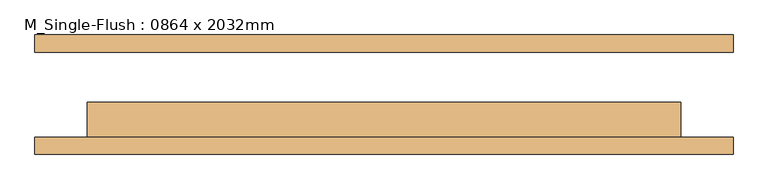
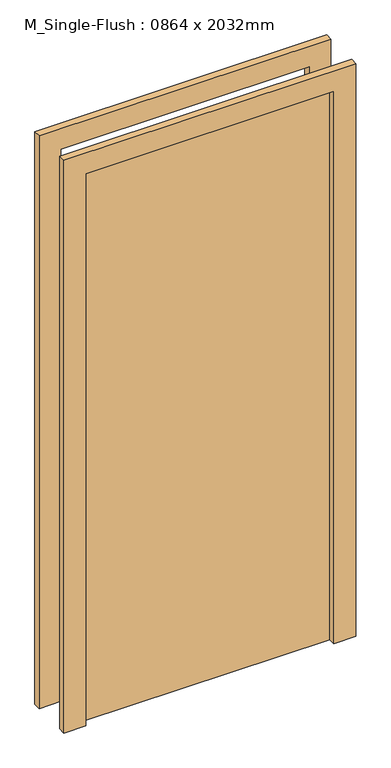
"""IFC4 building model written with IfcOpenShell, lengths in millimetres: door geometry, M_Single-Flush : 0864 x 2032mm."""

from ifc_helpers import new_model, si_unit, frame, origin, origin_with_axes, place, context, project, spatial, polyline, outline, extrude, source, transform, mapped, element, save


def m_single_flush_0864_x_2032mm_954ee019(model_context):
    return source(origin(), model_context, "Body", "SweptSolid", [
        extrude(outline(polyline([(2108.0, -508.0), (0.0, -508.0), (0.0, -432.0), (2032.0, -432.0), (2032.0, 432.0), (0.0, 432.0), (0.0, 508.0), (2108.0, 508.0), (2108.0, -508.0)])), frame((0.0, -87.0, 0.0), z_axis=(0.0, 1.0, 0.0), x_axis=(0.0, 0.0, 1.0)), (0.0, 0.0, 1.0), 25.0),
        extrude(outline(polyline([(2108.0, 508.0), (2108.0, -508.0), (0.0, -508.0), (0.0, -432.0), (2032.0, -432.0), (2032.0, 432.0), (0.0, 432.0), (0.0, 508.0), (2108.0, 508.0)])), frame((0.0, 62.0, 0.0), z_axis=(0.0, 1.0, 0.0), x_axis=(0.0, 0.0, 1.0)), (0.0, 0.0, 1.0), 25.0),
        extrude(outline(polyline([(432.0, -11.0), (432.0, -62.0), (-432.0, -62.0), (-432.0, -11.0), (432.0, -11.0)])), origin_with_axes(), (0.0, 0.0, 1.0), 2032.0),
    ])


if __name__ == "__main__":
    model = new_model("IFC4")
    model_context = context("Model", 3, world=origin())
    ifc_project = project(units=[si_unit("LENGTHUNIT", "METRE", prefix="MILLI")], contexts=[model_context])
    site = spatial("IfcSite", under=ifc_project)
    building = spatial("IfcBuilding", under=site)
    placement = place(None, origin())
    m_single_flush_0864_x_2032mm_shape = m_single_flush_0864_x_2032mm_954ee019(model_context)
    element("IfcDoor", 1, ObjectType="M_Single-Flush : 0864 x 2032mm", at=placement, inside=building, context=model_context, shape_type="MappedRepresentation", body=[
        mapped(m_single_flush_0864_x_2032mm_shape, transform((0.0, 0.0, 0.0), x_axis=(1.0, 0.0, 0.0), y_axis=(0.0, 1.0, 0.0), z_axis=(0.0, 0.0, 1.0))),
    ])
    save(model, "model.ifc")

# Revit data of these elements
# Type "M_Single-Flush : 0864 x 2032mm"
#   Manufacturer = "Manufacturer"
#   Type Mark = "32"
#   Construction Type = "Construction Type"
#   Fire Rating = "Fire Rating"
#   AccessibilityPerformance = "AccessibilityPerformance"
#   CodePerformance = "CodePerformance"
#   IsFireExit = "IsFireExit"
#   ConstructionType = "ConstructionType"
#   GlazingAreaFraction = "GlazingAreaFraction"
#   OperationType = "OperationType"
#   Area = "Area"
#   Color = "Color"
#   Constituents = "Constituents"
#   Features = "Features"
#   Finish = "Finish"
#   Grade = "Grade"
#   Material = "Material"
#   ModelReference = "ModelReference"
#   NominalHeight = "NominalHeight"
#   NominalLength = "NominalLength"
#   NominalWidth = "NominalWidth"
#   ProductionYear = "ProductionYear"
#   Reference = "Reference"
#   Shape = "Shape"
#   Size = "Size"
#   SustainabilityPerformance = "SustainabilityPerformance"
#   WarrantyDescription = "WarrantyDescription"
#   WarrantyDurationLabor = "WarrantyDurationLabor"
#   WarrantyDurationParts = "WarrantyDurationParts"
#   WarrantyGuarantorLabor = "WarrantyGuarantorLabor"
#   WarrantyGuarantorParts = "WarrantyGuarantorParts"
#   ExpectedLife = "ExpectedLife"
#   ReplacementCost = "ReplacementCost"
#   AssetAccountingType = "FIXED"
#   ModelLabel = "ModelLabel"
#   Thickness = 0.051 m
#   Height = 2.032 m
#   Trim Projection Ext = 0.025 m
#   Trim Projection Int = 0.025 m
#   Trim Width = 0.076 m
#   Width = 0.864 m
#   Door Material = Door - Panel
#   Frame Material = Door - Frame
#   Function = (empty or 0)
#   Wall Closure = (empty or 0)
# Element 1 (IfcDoor, "M_Single-Flush : 0864 x 2032mm")
#   Materials on its faces: "Door - Frame", "Door - Panel"
# Materials
#   "Door - Panel": class "Wood", colour RGB 210 159 95, transparency 0
#   "Door - Frame": class "Miscellaneous", colour RGB 118 70 51, transparency 0
